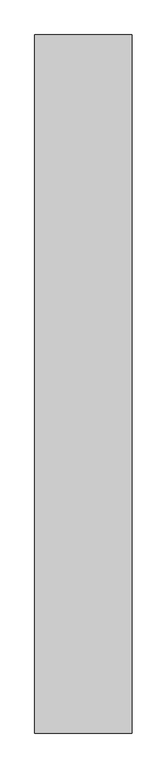
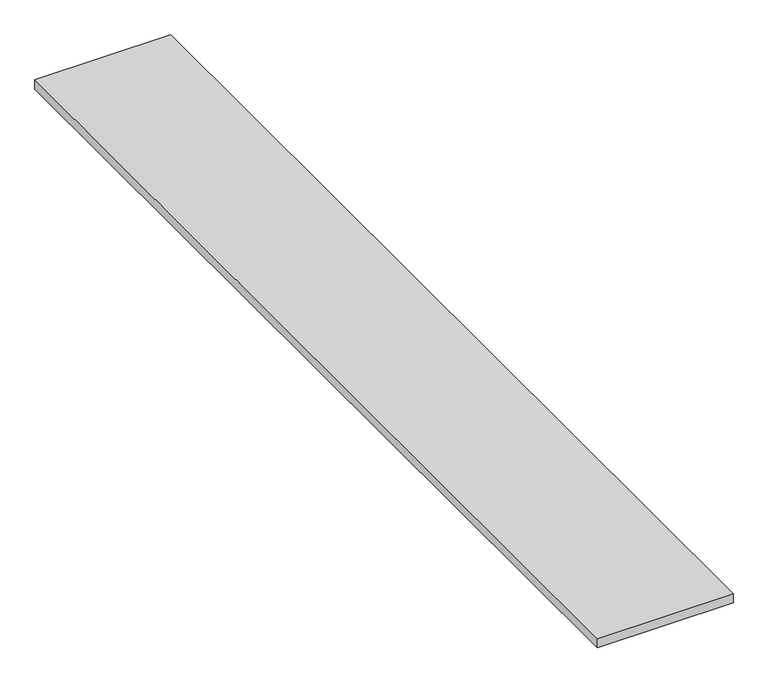
"""IFC4 building model written with IfcOpenShell, lengths in millimetres: furniture geometry, Furniture 2:Furniture 1:2369:Furniture 1:2369 : Furniture 2:Furniture 1:2369:300215 : Furniture 2:Furniture 1:2369:Furniture 1:2369 : Furniture 2:Furniture 1:2369:300215."""

from ifc_helpers import new_model, si_unit, frame, origin, place, context, project, spatial, polyline, outline, extrude, source, transform, mapped, element, save


def furniture_e357f16d(model_context):
    return source(origin(), model_context, "Body", "SweptSolid", [
        extrude(outline(polyline([(651443.7117239, -570612.3413841), (651443.7117239, -568059.6413841), (651799.3117239, -568059.6413841), (651799.3117239, -570612.3413841), (651443.7117239, -570612.3413841)])), frame((0.0, 0.0, 381.0), z_axis=(0.0, 0.0, 1.0), x_axis=(1.0, 0.0, 0.0)), (0.0, 0.0, 1.0), 25.4),
    ])


if __name__ == "__main__":
    model = new_model("IFC4")
    model_context = context("Model", 3, world=origin())
    ifc_project = project(units=[si_unit("LENGTHUNIT", "METRE", prefix="MILLI")], contexts=[model_context])
    site = spatial("IfcSite", under=ifc_project)
    building = spatial("IfcBuilding", under=site)
    placement = place(None, origin())
    furniture_shape = furniture_e357f16d(model_context)
    element("IfcFurniture", 1, ObjectType="Furniture 2:Furniture 1:2369:Furniture 1:2369 : Furniture 2:Furniture 1:2369:300215 : Furniture 2:Furniture 1:2369:Furniture 1:2369 : Furniture 2:Furniture 1:2369:300215", at=placement, inside=building, context=model_context, shape_type="MappedRepresentation", body=[
        mapped(furniture_shape, transform((0.0, 0.0, 0.0), x_axis=(1.0, 0.0, 0.0), y_axis=(0.0, 1.0, 0.0), z_axis=(0.0, 0.0, 1.0))),
    ])
    save(model, "model.ifc")

# Revit data of these elements
# Type "Furniture 2:Furniture 1:2369:Furniture 1:2369 : Furniture 2:Furniture 1:2369:300215 : Furniture 2:Furniture 1:2369:Furniture 1:2369 : Furniture 2:Furniture 1:2369:300215"
#   NameOverride = "Furniture 2:Furniture 1:2369:Furniture 1:2369 : Furniture 2:Furniture 1:2369:300215"
#   ObjectTypeOverride = "Furniture 1:2369 : Furniture 2:Furniture 1:2369"
#   Tag = "300215"
